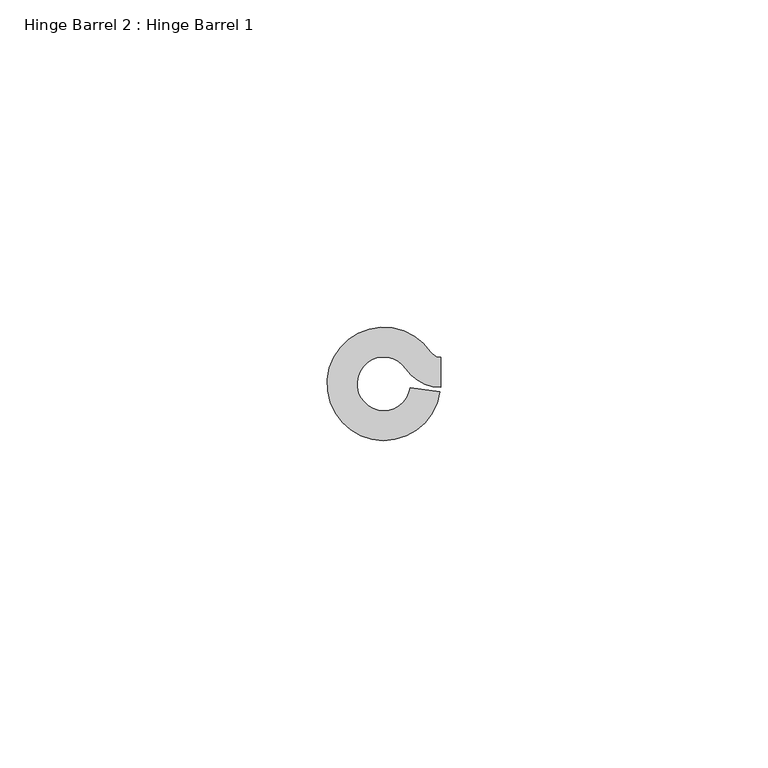
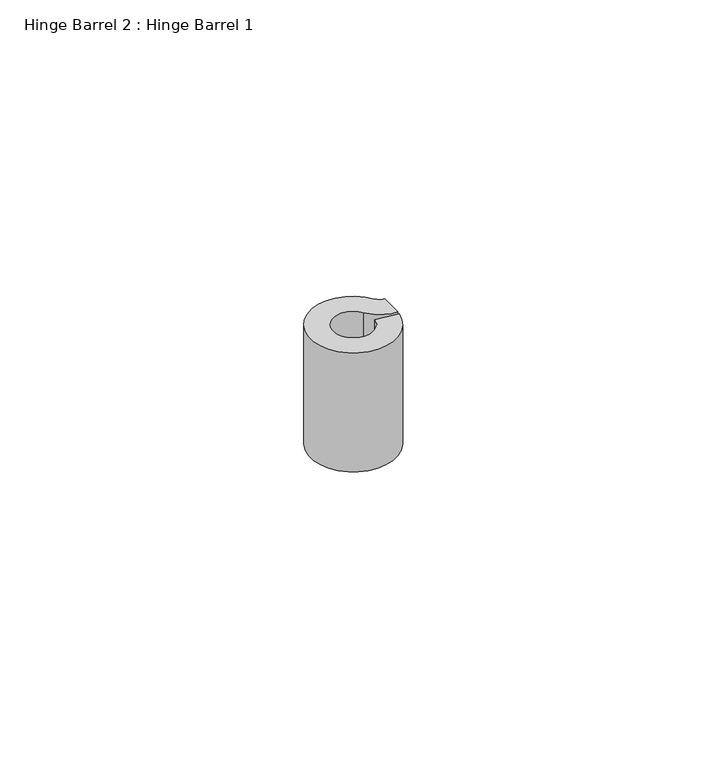
"""IFC4 building model written with IfcOpenShell, lengths in millimetres: proxy geometry, Hinge Barrel 2 : Hinge Barrel 1."""

from ifc_helpers import new_model, si_unit, point, frame, frame_2d, origin, place, context, project, spatial, polyline, circle_curve, trimmed, segment, composite_curve, outline, extrude, source, transform, mapped, element, save


def hinge_barrel_2_hinge_barrel_1_554cdc94(model_context):
    return source(origin(), model_context, "Body", "SweptSolid", [
        extrude(outline(composite_curve([segment(trimmed(circle_curve(frame_2d((587319.1320739, -531776.6049841)), 4.0894), [point((587322.5194669, -531774.3139665))], [point((587323.1821338, -531777.1708529))], True, "CARTESIAN"), True, "CONTINUOUS"), segment(polyline([(587323.1821338, -531777.1708529), (587327.7022899, -531777.8024028)]), True, "CONTINUOUS"), segment(trimmed(circle_curve(frame_2d((587319.1320739, -531776.6049841)), 8.6534625), [point((587327.7022899, -531777.8024028))], [point((587326.3000393, -531771.7570273))], False, "CARTESIAN"), True, "CONTINUOUS"), segment(trimmed(circle_curve(frame_2d((587327.8245257, -531770.7259615)), 1.8404226), [point((587326.3000393, -531771.7570273))], [point((587327.8245257, -531772.5663841))], True, "CARTESIAN"), True, "CONTINUOUS"), segment(polyline([(587327.8245257, -531772.5663841), (587327.8245257, -531777.1304466)]), True, "CONTINUOUS"), segment(trimmed(circle_curve(frame_2d((587327.8245257, -531770.7259615)), 6.4044851), [point((587327.8245257, -531777.1304466))], [point((587322.5194669, -531774.3139665))], False, "CARTESIAN"), True, "CONTINUOUS")], self_intersect=False)), frame((0.0, 0.0, 336.55), z_axis=(0.0, 0.0, 1.0), x_axis=(1.0, 0.0, 0.0)), (0.0, 0.0, 1.0), 25.4),
    ])


if __name__ == "__main__":
    model = new_model("IFC4")
    model_context = context("Model", 3, world=origin())
    ifc_project = project(units=[si_unit("LENGTHUNIT", "METRE", prefix="MILLI")], contexts=[model_context])
    site = spatial("IfcSite", under=ifc_project)
    building = spatial("IfcBuilding", under=site)
    placement = place(None, origin())
    hinge_barrel_2_hinge_barrel_1_shape = hinge_barrel_2_hinge_barrel_1_554cdc94(model_context)
    element("IfcBuildingElementProxy", 1, Name="Hinge Barrel 2 : Hinge Barrel 1", ObjectType="Hinge Barrel 2 : Hinge Barrel 1", at=placement, inside=building, context=model_context, shape_type="MappedRepresentation", body=[
        mapped(hinge_barrel_2_hinge_barrel_1_shape, transform((0.0, 0.0, 0.0), x_axis=(1.0, 0.0, 0.0), y_axis=(0.0, 1.0, 0.0), z_axis=(0.0, 0.0, 1.0))),
    ])
    save(model, "model.ifc")

# Revit data of these elements
# Element 1 (IfcBuildingElementProxy, "Hinge Barrel 2 : Hinge Barrel 1")
#   Materials on its faces: "6\"X6\" WELD-ON STL BUTT HINGE"
# Materials
#   "6\"X6\" WELD-ON STL BUTT HINGE": class "Metal", colour RGB 189 187 185, transparency 0, Description = "Carbon steel", Cost = 0
